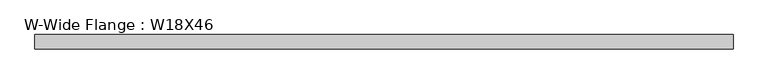
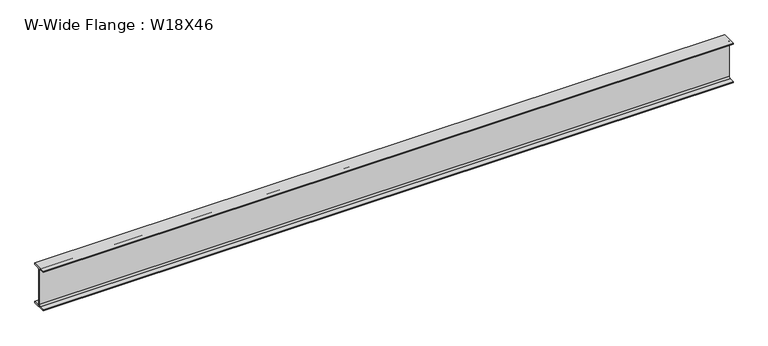
"""IFC4 building model written with IfcOpenShell, lengths in millimetres: beam geometry, W-Wide Flange : W18X46."""

import ifcopenshell
import ifcopenshell.guid

model = None  # the IFC model being written
_history = None  # IfcOwnerHistory: only IFC2X3 demands one
_inside = {}  # id of a spatial element -> (the spatial element, [elements in it])
_under = {}  # id of a project, library or spatial element -> (it, [spatial elements below it])
_declared = {}  # id of a project -> (the project, [libraries it declares])
_typed = {}  # id of a type object -> (the type object, [elements of that type])
_made_of = {}  # id of a material, layer set ... -> (it, [elements and type objects made of it])


def new_model(schema):
    """Start an empty IFC model of exactly this schema.

    Asked for "IFC4X3", IfcOpenShell would pick the latest addendum, in which some entities
    have other attributes; the version numbers below select the first issue.
    IFC2X3 requires an IfcOwnerHistory on every rooted entity: one is made here for all.
    """
    global model, _history
    if schema == "IFC4X3":
        model = ifcopenshell.file(schema_version=(4, 3, 0, 0))
    else:
        model = ifcopenshell.file(schema=schema)
    _inside.clear()
    _under.clear()
    _declared.clear()
    _typed.clear()
    _made_of.clear()
    _history = None
    if model.schema == "IFC2X3":
        org = make("IfcOrganization", Name="unknown")
        user = make(
            "IfcPersonAndOrganization",
            ThePerson=make("IfcPerson", FamilyName="unknown"),
            TheOrganization=org,
        )
        app = make(
            "IfcApplication",
            ApplicationDeveloper=org,
            Version="unknown",
            ApplicationFullName="unknown",
            ApplicationIdentifier="unknown",
        )
        _history = make(
            "IfcOwnerHistory",
            OwningUser=user,
            OwningApplication=app,
            ChangeAction="ADDED",
            CreationDate=0,
        )
    return model


def make(cls, **values):
    """One entity of the class cls with the attributes given. An attribute that is None is left unset."""
    return model.create_entity(
        cls, **{name: value for name, value in values.items() if value is not None}
    )


def rooted(cls, **values):
    """An entity with a GlobalId (a new one), such as an element, a storey or a relation."""
    return make(cls, GlobalId=ifcopenshell.guid.new(), OwnerHistory=_history, **values)


def si_unit(unit_type, name, prefix=None):
    """IfcSIUnit, for example si_unit("LENGTHUNIT", "METRE", prefix="MILLI")."""
    return make("IfcSIUnit", UnitType=unit_type, Prefix=prefix, Name=name)


def assignment(units):
    """IfcUnitAssignment: the units of a project."""
    return None if units is None else make("IfcUnitAssignment", Units=units)


def point(xyz):
    """IfcCartesianPoint."""
    return None if xyz is None else make("IfcCartesianPoint", Coordinates=xyz)


def direction(xyz):
    """IfcDirection."""
    return None if xyz is None else make("IfcDirection", DirectionRatios=xyz)


def frame(location, z_axis=None, x_axis=None):
    """IfcAxis2Placement3D, a coordinate frame: its origin and axes. An axis left out is left unset."""
    return make(
        "IfcAxis2Placement3D",
        Location=point(location),
        Axis=direction(z_axis),
        RefDirection=direction(x_axis),
    )


def frame_2d(location, x_axis=None):
    """IfcAxis2Placement2D, a coordinate frame in the plane: its origin and x axis."""
    return make(
        "IfcAxis2Placement2D", Location=point(location), RefDirection=direction(x_axis)
    )


def origin():
    """The frame at (0, 0, 0) with its axes left unset."""
    return frame((0.0, 0.0, 0.0))


def place(relative_to, where):
    """IfcLocalPlacement: puts the frame where relative to a parent placement (None: the world)."""
    return make(
        "IfcLocalPlacement", PlacementRelTo=relative_to, RelativePlacement=where
    )


def context(
    kind, dimensions, precision=None, world=None, true_north=None, identifier=None
):
    """IfcGeometricRepresentationContext, for example the 3D "Model" context."""
    return make(
        "IfcGeometricRepresentationContext",
        ContextIdentifier=identifier,
        ContextType=kind,
        CoordinateSpaceDimension=dimensions,
        Precision=precision,
        WorldCoordinateSystem=world,
        TrueNorth=true_north,
    )


def project(units=None, contexts=None):
    """IfcProject with its units and contexts."""
    return rooted(
        "IfcProject",
        Name="project",
        RepresentationContexts=contexts,
        UnitsInContext=assignment(units),
    )


def spatial(cls, under=None, at=None, **own):
    """A site, building, storey or space (cls), placed at a placement, below another one or the project."""
    s = rooted(cls, ObjectPlacement=at, **own)
    if under is not None:
        _under.setdefault(under.id(), (under, []))[1].append(s)
    return s


def polyline(points):
    """IfcPolyline through the points."""
    return make("IfcPolyline", Points=[point(p) for p in points])


def circle_curve(where, radius):
    """IfcCircle in the frame where."""
    return make("IfcCircle", Position=where, Radius=radius)


def trimmed(basis, trim1, trim2, sense, master):
    """IfcTrimmedCurve: the piece of a basis curve between two trims."""
    return make(
        "IfcTrimmedCurve",
        BasisCurve=basis,
        Trim1=trim1,
        Trim2=trim2,
        SenseAgreement=sense,
        MasterRepresentation=master,
    )


def segment(curve, same_sense, transition):
    """IfcCompositeCurveSegment."""
    return make(
        "IfcCompositeCurveSegment",
        Transition=transition,
        SameSense=same_sense,
        ParentCurve=curve,
    )


def composite_curve(segments, self_intersect=None):
    """IfcCompositeCurve: segments joined end to end."""
    return make("IfcCompositeCurve", Segments=segments, SelfIntersect=self_intersect)


def outline(outer, holes=None, kind="AREA"):
    """IfcArbitraryClosedProfileDef: a profile drawn as a closed curve; with holes, ...WithVoids."""
    if holes is None:
        return make("IfcArbitraryClosedProfileDef", ProfileType=kind, OuterCurve=outer)
    return make(
        "IfcArbitraryProfileDefWithVoids",
        ProfileType=kind,
        OuterCurve=outer,
        InnerCurves=holes,
    )


def extrude(swept, where, along, depth):
    """IfcExtrudedAreaSolid: the profile swept, set in the frame where, extruded along a direction by depth."""
    return make(
        "IfcExtrudedAreaSolid",
        SweptArea=swept,
        Position=where,
        ExtrudedDirection=direction(along),
        Depth=depth,
    )


def shape(context_of_items, identifier, shape_type, items):
    """IfcShapeRepresentation: the items that make up one representation, for example the "Body"."""
    return make(
        "IfcShapeRepresentation",
        ContextOfItems=context_of_items,
        RepresentationIdentifier=identifier,
        RepresentationType=shape_type,
        Items=items,
    )


def source(mapping_origin, context_of_items, identifier, shape_type, items):
    """IfcRepresentationMap: a shape defined once, which mapped items show again and again."""
    return make(
        "IfcRepresentationMap",
        MappingOrigin=mapping_origin,
        MappedRepresentation=shape(context_of_items, identifier, shape_type, items),
    )


def transform(
    local_origin,
    x_axis=None,
    y_axis=None,
    z_axis=None,
    scale=None,
    scale2=None,
    scale3=None,
    uniform=True,
):
    """IfcCartesianTransformationOperator3D, or its non-uniform kind. x_axis, y_axis, z_axis: its Axis1, 2, 3."""
    if uniform:
        return make(
            "IfcCartesianTransformationOperator3D",
            Axis1=direction(x_axis),
            Axis2=direction(y_axis),
            LocalOrigin=point(local_origin),
            Scale=scale,
            Axis3=direction(z_axis),
        )
    return make(
        "IfcCartesianTransformationOperator3DnonUniform",
        Axis1=direction(x_axis),
        Axis2=direction(y_axis),
        LocalOrigin=point(local_origin),
        Scale=scale,
        Axis3=direction(z_axis),
        Scale2=scale2,
        Scale3=scale3,
    )


def mapped(mapping_source, mapping_target):
    """IfcMappedItem: shows the shape of a source again, moved by a transform."""
    return make(
        "IfcMappedItem", MappingSource=mapping_source, MappingTarget=mapping_target
    )


def made_of(thing, what):
    """Note that an element or type object is made of a material, layer set ...; save() writes the relation."""
    if what is not None:
        _made_of.setdefault(what.id(), (what, []))[1].append(thing)
    return thing


def element(
    cls,
    number,
    at=None,
    inside=None,
    cuts=None,
    type_object=None,
    material=None,
    context=None,
    identifier="Body",
    shape_type=None,
    held_by="IfcProductDefinitionShape",
    body=None,
    shapes=None,
    **own,
):
    """One element of the class cls, such as IfcWall. Its Tag is "e" and its number.

    at: its placement. inside: the storey or other place that contains it. cuts: it is an
    opening in that element (IfcRelVoidsElement). A single representation is given by context,
    identifier, shape_type and body (its items); several are given by shapes. held_by: the class
    of the entity that holds the representations. save() writes the other relations.
    """
    e = rooted(cls, Tag="e%d" % number, ObjectPlacement=at, **own)
    if body is not None:
        shapes = [shape(context, identifier, shape_type, body)]
    if shapes is not None:
        e.Representation = make(held_by, Representations=shapes)
    if inside is not None:
        _inside.setdefault(inside.id(), (inside, []))[1].append(e)
    if cuts is not None:
        rooted(
            "IfcRelVoidsElement", RelatingBuildingElement=cuts, RelatedOpeningElement=e
        )
    if type_object is not None:
        _typed.setdefault(type_object.id(), (type_object, []))[1].append(e)
    return made_of(e, material)


def aggregate(whole, parts):
    """IfcRelAggregates: a whole, such as a stair, and the parts it consists of."""
    return rooted("IfcRelAggregates", RelatingObject=whole, RelatedObjects=parts)


def save(model, path):
    """Write the relations noted so far, then the file.

    IfcRelAggregates (storeys below a building ...), IfcRelContainedInSpatialStructure (elements
    in a storey), IfcRelDefinesByType, IfcRelAssociatesMaterial and IfcRelDeclares: one each for
    every whole, place, type object, material and project.
    """
    for whole, parts in _under.values():
        aggregate(whole, parts)
    for where, things in _inside.values():
        rooted(
            "IfcRelContainedInSpatialStructure",
            RelatedElements=things,
            RelatingStructure=where,
        )
    for kind, things in _typed.values():
        rooted("IfcRelDefinesByType", RelatedObjects=things, RelatingType=kind)
    for what, things in _made_of.values():
        rooted("IfcRelAssociatesMaterial", RelatedObjects=things, RelatingMaterial=what)
    for by, libraries in _declared.values():
        rooted("IfcRelDeclares", RelatingContext=by, RelatedDefinitions=libraries)
    model.write(path)


def w_wide_flange_w18x46_8f6cf0fd(model_context):
    return source(origin(), model_context, "Body", "SweptSolid", [
        extrude(outline(composite_curve([segment(polyline([(76.962, -214.503), (76.962, -229.87), (-76.962, -229.87), (-76.962, -214.503), (-20.955, -214.503)]), True, "CONTINUOUS"), segment(trimmed(circle_curve(frame_2d((-20.955, -198.12)), 16.383), [point((-20.955, -214.503))], [point((-4.572, -198.12))], True, "CARTESIAN"), True, "CONTINUOUS"), segment(polyline([(-4.572, -198.12), (-4.572, 198.12)]), True, "CONTINUOUS"), segment(trimmed(circle_curve(frame_2d((-20.955, 198.12)), 16.383), [point((-4.572, 198.12))], [point((-20.955, 214.503))], True, "CARTESIAN"), True, "CONTINUOUS"), segment(polyline([(-20.955, 214.503), (-76.962, 214.503), (-76.962, 229.87), (76.962, 229.87), (76.962, 214.503), (20.955, 214.503)]), True, "CONTINUOUS"), segment(trimmed(circle_curve(frame_2d((20.955, 198.12)), 16.383), [point((20.955, 214.503))], [point((4.572, 198.12))], True, "CARTESIAN"), True, "CONTINUOUS"), segment(polyline([(4.572, 198.12), (4.572, -198.12)]), True, "CONTINUOUS"), segment(trimmed(circle_curve(frame_2d((20.955, -198.12)), 16.383), [point((4.572, -198.12))], [point((20.955, -214.503))], True, "CARTESIAN"), True, "CONTINUOUS"), segment(polyline([(20.955, -214.503), (76.962, -214.503)]), True, "CONTINUOUS")], self_intersect=False)), frame((-3764.7066406, 0.0, 0.0), z_axis=(1.0, 0.0, 0.0), x_axis=(0.0, 1.0, 0.0)), (0.0, 0.0, 1.0), 7529.4132813),
    ])


if __name__ == "__main__":
    model = new_model("IFC4")
    model_context = context("Model", 3, world=origin())
    ifc_project = project(units=[si_unit("LENGTHUNIT", "METRE", prefix="MILLI")], contexts=[model_context])
    site = spatial("IfcSite", under=ifc_project)
    building = spatial("IfcBuilding", under=site)
    placement = place(None, origin())
    w_wide_flange_w18x46_shape = w_wide_flange_w18x46_8f6cf0fd(model_context)
    element("IfcBeam", 1, ObjectType="W-Wide Flange : W18X46", at=placement, inside=building, context=model_context, shape_type="MappedRepresentation", body=[
        mapped(w_wide_flange_w18x46_shape, transform((0.0, 0.0, 0.0), x_axis=(1.0, 0.0, 0.0), y_axis=(0.0, 1.0, 0.0), z_axis=(0.0, 0.0, 1.0))),
    ])
    save(model, "model.ifc")

# Revit data of these elements
# Type "W-Wide Flange : W18X46"
#   Assembly Code = "B10"
#   W = 46
#   Length [instance default] = 1524 mm
#   bf = 153.924 mm
#   d = 459.74 mm
#   k = 31.75 mm
#   k2 = 16.383 mm
#   tf = 15.367 mm
#   tw = 9.144 mm
#   A = 0.00870966 m²
#   Structural Material [instance default] = Steel ASTM A992
# Element 1 (IfcBeam, "W-Wide Flange : W18X46")
#   Structural Material = Aluminum, Anodized Red
#   Materials on its faces: "Aluminum, Anodized Red"
# Materials
#   "Steel ASTM A992": class "Metal", colour RGB 128 0 0, transparency 0, Description = "Structural steel 50ksi", Cost = 0
#   "Aluminum, Anodized Red": class "Metal", colour RGB 120 120 120, transparency 0, Description = "Anodized aluminum, red", Cost = 0
